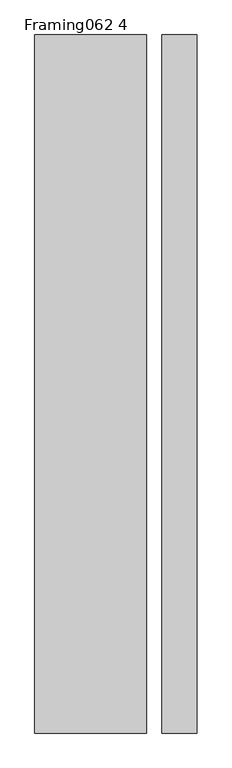
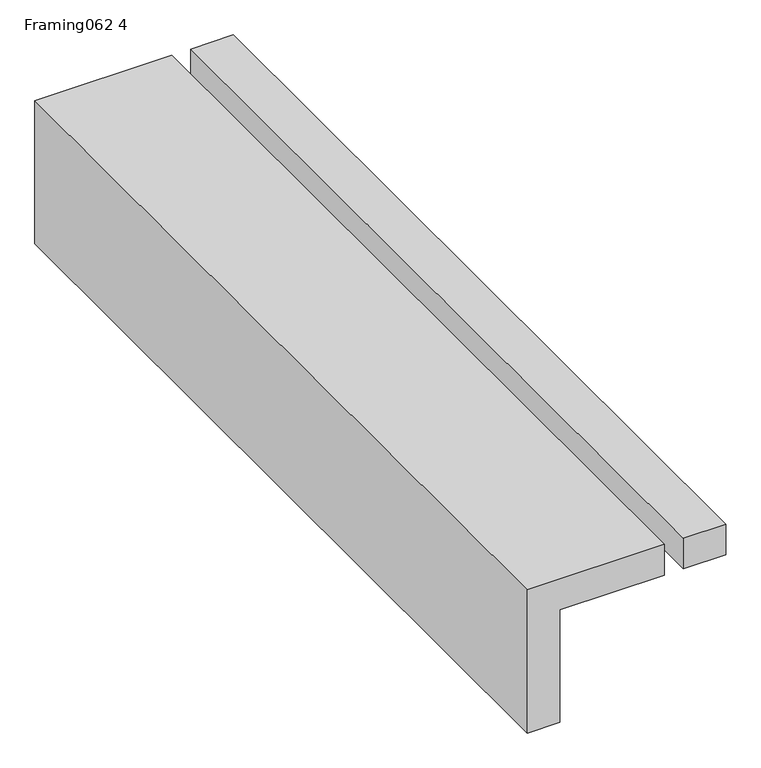
"""IFC4 building model written with IfcOpenShell, lengths in millimetres: proxy geometry, Framing062 4 : Framing062 15035."""

from ifc_helpers import new_model, si_unit, frame, origin, place, context, project, spatial, polyline, outline, extrude, source, transform, mapped, element, save


def framing062_4_cbcbbf25(model_context):
    return source(origin(), model_context, "Body", "SweptSolid", [
        extrude(outline(polyline([(42134.105552, -863.3885697), (42413.2036692, -863.3885697), (42413.2036692, -618.6019086), (42489.4036692, -618.6019086), (42489.4036692, -939.5885697), (42134.105552, -939.5885697), (42134.105552, -863.3885697)])), frame((0.0, -1052.8906574, 0.0), z_axis=(0.0, 1.0, 0.0), x_axis=(0.0, 0.0, 1.0)), (0.0, 0.0, 1.0), 2000.0),
        extrude(outline(polyline([(-474.2526923, -1052.8906574), (-574.1519086, -1052.8906574), (-574.1519086, 947.1093426), (-474.2526923, 947.1093426), (-474.2526923, -1052.8906574)])), frame((0.0, 0.0, 42413.2036692), z_axis=(0.0, 0.0, 1.0), x_axis=(1.0, 0.0, 0.0)), (0.0, 0.0, 1.0), 76.2),
    ])


if __name__ == "__main__":
    model = new_model("IFC4")
    model_context = context("Model", 3, world=origin())
    ifc_project = project(units=[si_unit("LENGTHUNIT", "METRE", prefix="MILLI")], contexts=[model_context])
    site = spatial("IfcSite", under=ifc_project)
    building = spatial("IfcBuilding", under=site)
    placement = place(None, origin())
    framing062_4_shape = framing062_4_cbcbbf25(model_context)
    element("IfcBuildingElementProxy", 1, Name="Framing062 4 : Framing062 15035", ObjectType="Framing062 4 : Framing062 15035", at=placement, inside=building, context=model_context, shape_type="MappedRepresentation", body=[
        mapped(framing062_4_shape, transform((0.0, 0.0, 0.0), x_axis=(1.0, 0.0, 0.0), y_axis=(0.0, 1.0, 0.0), z_axis=(0.0, 0.0, 1.0))),
    ])
    save(model, "model.ifc")

# Revit data of these elements
# Type "Framing062 4 : Framing062 15035"
#   NameOverride = "Framing062"
# Element 1 (IfcBuildingElementProxy, "Framing062 4 : Framing062 15035")
#   Materials on its faces: "3\" POLYURETHANE SPRAY FOAM UNDER ROOF SUBSTRATE"
# Materials
#   "3\" POLYURETHANE SPRAY FOAM UNDER ROOF SUBSTRATE": class "Unassigned", colour RGB 210 164 194, transparency 0, Cost = 0
